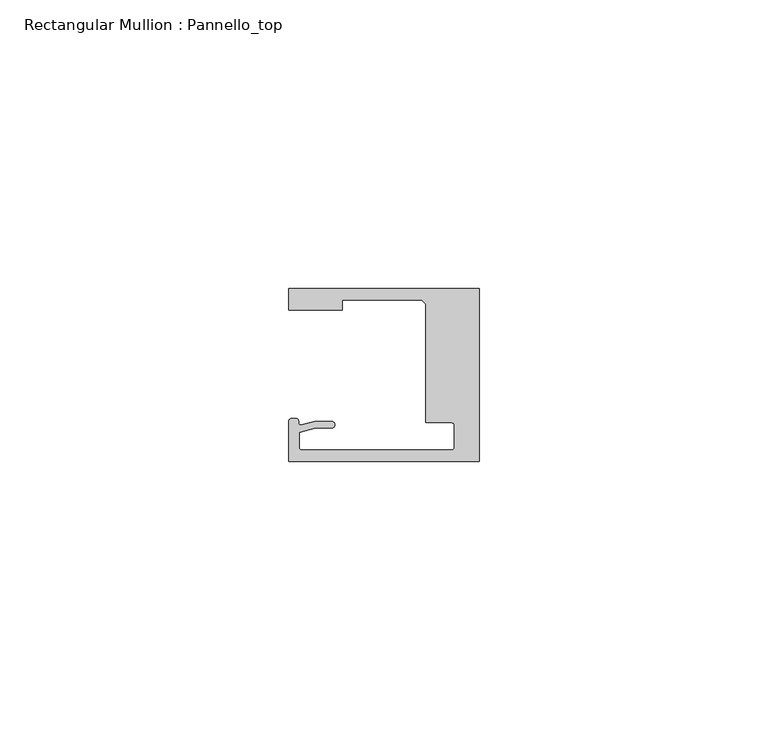
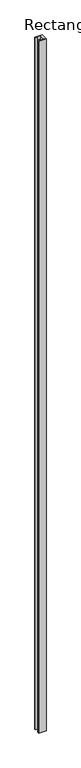
"""IFC4 building model written with IfcOpenShell, lengths in millimetres: member geometry, Rectangular Mullion : Pannello_top."""

from ifc_helpers import new_model, si_unit, frame, origin, place, context, project, spatial, polyline, circle_curve, source, transform, mapped, element, save
from ifc_brep_helpers import plane_surface, cylinder_surface, revolved_surface, extruded_surface, spline_curve, advanced_brep


def rectangular_mullion_pannello_top_1276d198(model_context):
    return source(origin(), model_context, "Body", "AdvancedBrep", [
        advanced_brep(
        [(-33.0, 15.0, 0.0), (-33.0, 11.3000004, 0.0), (-23.700041, 11.3000004, 0.0), (-23.700041, 13.0000004, 0.0), (-10.0000103, 13.0000004, 0.0), (-9.2999726, 12.2999849, 0.0), (-9.2999726, -8.2500595, 0.0), (-4.7999726, -8.2500595, 0.0), (-4.2999726, -8.7500595, 0.0), (-4.2999726, -12.50001, 0.0), (-4.7999726, -13.00001, 0.0), (-30.69998, -13.00001, 0.0), (-31.19998, -12.50001, 0.0), (-31.19998, -9.9657591, 0.0), (-28.3419477, -9.1999523, 0.0), (-25.59998, -9.1999523, 0.0), (-25.59998, -7.9999523, 0.0), (-28.4999305, -7.9999523, 0.0), (-30.9223017, -8.6490241, 0.0), (-33.0000135, -8.0000472, 0.0), (-33.0000135, -15.0, 0.0), (0.0, -15.0, 0.0), (0.0, 15.0, 0.0), (-33.0, 15.0, -3313.9999729), (0.0, 15.0, -3313.9999729), (0.0, -15.0, -3313.9999729), (-33.0000135, -15.0, -3313.9999729), (-33.0000135, -8.0000472, -3313.9999729), (-30.9223017, -8.6490241, -3313.9999729), (-28.4999305, -7.9999523, -3313.9999729), (-25.59998, -7.9999523, -3313.9999729), (-25.59998, -9.1999523, -3313.9999729), (-28.3419477, -9.1999523, -3313.9999729), (-31.19998, -9.9657591, -3313.9999729), (-31.19998, -12.50001, -3313.9999729), (-30.69998, -13.00001, -3313.9999729), (-4.7999726, -13.00001, -3313.9999729), (-4.2999726, -12.50001, -3313.9999729), (-4.2999726, -8.7500595, -3313.9999729), (-4.7999726, -8.2500595, -3313.9999729), (-9.2999726, -8.2500595, -3313.9999729), (-9.2999726, 12.2999849, -3313.9999729), (-10.0000103, 13.0000004, -3313.9999729), (-23.700041, 13.0000004, -3313.9999729), (-23.700041, 11.3000004, -3313.9999729), (-33.0, 11.3000004, -3313.9999729)],
        [
            (0, 1),
            (1, 2),
            (2, 3),
            (3, 4),
            (4, 5),
            (5, 6),
            (6, 7),
            (7, 8, circle_curve(frame((-4.7999726, -8.7500595, 0.0), z_axis=(0.0, 0.0, -1.0), x_axis=(0.0, 1.0, 0.0)), 0.5)),
            (8, 9),
            (9, 10, circle_curve(frame((-4.7999726, -12.50001, 0.0), z_axis=(0.0, 0.0, -1.0), x_axis=(1.0, 0.0, 0.0)), 0.5)),
            (10, 11),
            (11, 12, circle_curve(frame((-30.69998, -12.50001, 0.0), z_axis=(0.0, 0.0, -1.0), x_axis=(0.0, -1.0, 0.0)), 0.5)),
            (12, 13),
            (13, 14),
            (14, 15),
            (15, 16, circle_curve(frame((-25.59998, -8.5999523, 0.0), z_axis=(0.0, 0.0, 1.0), x_axis=(0.0, -1.0, 0.0)), 0.6)),
            (16, 17),
            (17, 18),
            (18, 19, spline_curve(3, [(-30.9223017, -8.6490241, 0.0), (-31.312054066, -8.717747958, 0.0), (-31.298563602, -8.366228555, 0.0), (-31.305645054, -7.690065204, 0.0), (-31.357433266, -7.563996614, 0.0), (-32.262327879, -7.456527435, 0.0), (-33.0000135, -7.457047519, 0.0), (-33.0000135, -8.0000472, 0.0)], [4, 2, 2, 4], [0.0, 0.001840817752199412, 0.004996616814974408, 0.007702013405570312])),
            (19, 20),
            (20, 21),
            (21, 22),
            (22, 0),
            (23, 24),
            (24, 25),
            (25, 26),
            (26, 27),
            (27, 28, spline_curve(3, [(-33.0000135, -8.0000472, -3313.9999729), (-33.0000135, -7.457047519, -3313.9999729), (-32.262327879, -7.456527435, -3313.9999729), (-31.357433266, -7.563996614, -3313.9999729), (-31.305645054, -7.690065204, -3313.9999729), (-31.298563602, -8.366228555, -3313.9999729), (-31.312054066, -8.717747958, -3313.9999729), (-30.9223017, -8.6490241, -3313.9999729)], [4, 2, 2, 4], [0.0, 0.0027053965905959043, 0.0058611956533709, 0.007702013405570312])),
            (28, 29),
            (29, 30),
            (30, 31, circle_curve(frame((-25.59998, -8.5999523, -3313.9999729), z_axis=(0.0, 0.0, -1.0), x_axis=(0.0, -1.0, 0.0)), 0.6)),
            (31, 32),
            (32, 33),
            (33, 34),
            (34, 35, circle_curve(frame((-30.69998, -12.50001, -3313.9999729), z_axis=(0.0, 0.0, 1.0), x_axis=(0.0, -1.0, 0.0)), 0.5)),
            (35, 36),
            (36, 37, circle_curve(frame((-4.7999726, -12.50001, -3313.9999729), z_axis=(0.0, 0.0, 1.0), x_axis=(1.0, 0.0, 0.0)), 0.5)),
            (37, 38),
            (38, 39, circle_curve(frame((-4.7999726, -8.7500595, -3313.9999729), z_axis=(0.0, 0.0, 1.0), x_axis=(0.0, 1.0, 0.0)), 0.5)),
            (39, 40),
            (40, 41),
            (41, 42),
            (42, 43),
            (43, 44),
            (44, 45),
            (45, 23),
            (0, 23),
            (45, 1),
            (44, 2),
            (43, 3),
            (42, 4),
            (41, 5),
            (40, 6),
            (39, 7),
            (38, 8),
            (37, 9),
            (36, 10),
            (35, 11),
            (34, 12),
            (33, 13),
            (32, 14),
            (31, 15),
            (30, 16),
            (29, 17),
            (28, 18),
            (27, 19),
            (26, 20),
            (25, 21),
            (24, 22),
        ],
        [
            plane_surface(frame((0.0, -36.2491502, 0.0), z_axis=(0.0, 0.0, 1.0), x_axis=(-1.0, 0.0, 0.0))),
            plane_surface(frame((0.0, -36.2491502, -3313.9999729), z_axis=(0.0, 0.0, -1.0), x_axis=(-1.0, 0.0, 0.0))),
            plane_surface(frame((-33.0, 15.0, 0.0), z_axis=(-1.0, 0.0, 0.0), x_axis=(0.0, 0.0, -1.0))),
            plane_surface(frame((-33.0, 11.3000004, 0.0), z_axis=(0.0, -1.0, 0.0), x_axis=(0.0, 0.0, -1.0))),
            plane_surface(frame((-23.700041, 11.3000004, 0.0), z_axis=(1.0, 0.0, 0.0), x_axis=(0.0, 0.0, -1.0))),
            plane_surface(frame((-23.700041, 13.0000004, 0.0), z_axis=(0.0, -1.0, 0.0), x_axis=(0.0, 0.0, -1.0))),
            plane_surface(frame((-10.0000103, 13.0000004, 0.0), z_axis=(-0.7070955486277984, -0.7071180135668678, 0.0), x_axis=(0.0, 0.0, -1.0))),
            plane_surface(frame((-9.2999726, 12.2999849, 0.0), z_axis=(-1.0, 0.0, 0.0), x_axis=(0.0, 0.0, -1.0))),
            plane_surface(frame((-9.2999726, -8.2500595, 0.0), z_axis=(0.0, -1.0, 0.0), x_axis=(0.0, 0.0, -1.0))),
            revolved_surface(polyline([(-4.7999726, -8.2500595, -3313.9999729), (-4.7999726, -8.2500595, 0.0)]), (-4.7999726, -8.7500595, 0.0), (0.0, 0.0, -1.0)),
            plane_surface(frame((-4.2999726, -8.7500595, 0.0), z_axis=(-1.0, 0.0, 0.0), x_axis=(0.0, 0.0, -1.0))),
            revolved_surface(polyline([(-4.2999726, -12.50001, -3313.9999729), (-4.2999726, -12.50001, 0.0)]), (-4.7999726, -12.50001, 0.0), (0.0, 0.0, -1.0)),
            plane_surface(frame((-4.7999726, -13.00001, 0.0), z_axis=(0.0, 1.0, 0.0), x_axis=(0.0, 0.0, -1.0))),
            revolved_surface(polyline([(-30.69998, -13.00001, -3313.9999729), (-30.69998, -13.00001, 0.0)]), (-30.69998, -12.50001, 0.0), (0.0, 0.0, -1.0)),
            plane_surface(frame((-31.19998, -12.50001, 0.0), z_axis=(1.0, 0.0, 0.0), x_axis=(0.0, 0.0, -1.0))),
            plane_surface(frame((-31.19998, -9.9657591, 0.0), z_axis=(0.25881883204288636, -0.9659258833782002, 0.0), x_axis=(0.0, 0.0, -1.0))),
            plane_surface(frame((-28.3419477, -9.1999523, 0.0), z_axis=(0.0, -1.0, 0.0), x_axis=(0.0, 0.0, -1.0))),
            cylinder_surface(frame((-25.59998, -8.5999523, 0.0), z_axis=(0.0, 0.0, 1.0), x_axis=(0.0, -1.0, 0.0)), 0.6),
            plane_surface(frame((-25.59998, -7.9999523, 0.0), z_axis=(0.0, 1.0, 0.0), x_axis=(0.0, 0.0, -1.0))),
            plane_surface(frame((-28.4999305, -7.9999523, 0.0), z_axis=(-0.25881883200192934, 0.9659258833891746, 0.0), x_axis=(0.0, 0.0, -1.0))),
            extruded_surface(spline_curve(3, [(-30.9223017, -8.6490241, -3313.9999729), (-31.312054066, -8.717747958, -3313.9999729), (-31.298563602, -8.366228555, -3313.9999729), (-31.305645054, -7.690065204, -3313.9999729), (-31.357433266, -7.563996614, -3313.9999729), (-32.262327879, -7.456527435, -3313.9999729), (-33.0000135, -7.457047519, -3313.9999729), (-33.0000135, -8.0000472, -3313.9999729)], [4, 2, 2, 4], [0.0, 0.001840817752199412, 0.004996616814974408, 0.007702013405570312]), (0.0, 0.0, 3313.9999729), 3313.9999729),
            plane_surface(frame((-33.0000135, -8.0000472, 0.0), z_axis=(-1.0, 0.0, 0.0), x_axis=(0.0, 0.0, -1.0))),
            plane_surface(frame((-33.0000135, -15.0, 0.0), z_axis=(0.0, -1.0, 0.0), x_axis=(0.0, 0.0, -1.0))),
            plane_surface(frame((0.0, -15.0, 0.0), z_axis=(1.0, 0.0, 0.0), x_axis=(0.0, 0.0, -1.0))),
            plane_surface(frame((0.0, 15.0, 0.0), z_axis=(0.0, 1.0, 0.0), x_axis=(0.0, 0.0, -1.0))),
        ],
        [
            (0, [[1, 2, 3, 4, 5, 6, 7, 8, 9, 10, 11, 12, 13, 14, 15, 16, 17, 18, 19, 20, 21, 22, 23]]),
            (1, [[24, 25, 26, 27, 28, 29, 30, 31, 32, 33, 34, 35, 36, 37, 38, 39, 40, 41, 42, 43, 44, 45, 46]]),
            (2, [[-1, 47, -46, 48]]),
            (3, [[-2, -48, -45, 49]]),
            (4, [[-3, -49, -44, 50]]),
            (5, [[-4, -50, -43, 51]]),
            (6, [[-5, -51, -42, 52]]),
            (7, [[-6, -52, -41, 53]]),
            (8, [[-7, -53, -40, 54]]),
            (9, [[-8, -54, -39, 55]]),
            (10, [[-9, -55, -38, 56]]),
            (11, [[-10, -56, -37, 57]]),
            (12, [[-11, -57, -36, 58]]),
            (13, [[-12, -58, -35, 59]]),
            (14, [[-13, -59, -34, 60]]),
            (15, [[-14, -60, -33, 61]]),
            (16, [[-15, -61, -32, 62]]),
            (17, [[-16, -62, -31, 63]]),
            (18, [[-17, -63, -30, 64]]),
            (19, [[-18, -64, -29, 65]]),
            (20, [[-19, -65, -28, 66]]),
            (21, [[-20, -66, -27, 67]]),
            (22, [[-21, -67, -26, 68]]),
            (23, [[-22, -68, -25, 69]]),
            (24, [[-23, -69, -24, -47]]),
        ],
    ),
    ])


if __name__ == "__main__":
    model = new_model("IFC4")
    model_context = context("Model", 3, world=origin())
    ifc_project = project(units=[si_unit("LENGTHUNIT", "METRE", prefix="MILLI")], contexts=[model_context])
    site = spatial("IfcSite", under=ifc_project)
    building = spatial("IfcBuilding", under=site)
    placement = place(None, origin())
    rectangular_mullion_pannello_top_shape = rectangular_mullion_pannello_top_1276d198(model_context)
    element("IfcMember", 1, ObjectType="Rectangular Mullion : Pannello_top", at=placement, inside=building, context=model_context, shape_type="MappedRepresentation", body=[
        mapped(rectangular_mullion_pannello_top_shape, transform((0.0, 0.0, 0.0), x_axis=(1.0, 0.0, 0.0), y_axis=(0.0, 1.0, 0.0), z_axis=(0.0, 0.0, 1.0))),
    ])
    save(model, "model.ifc")

# Revit data of these elements
# Type "Rectangular Mullion : Pannello_top"
#   built-in parameter 1007322 = 0.0984252 (stored number, unit not read)
#   built-in parameter 1007321 = 0 (stored number, unit not read)
#   built-in parameter 1007320 = 0.0305117 (stored number, unit not read)
